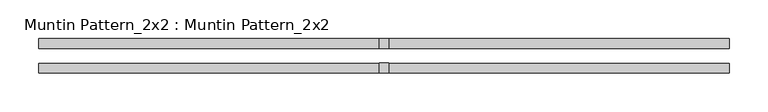
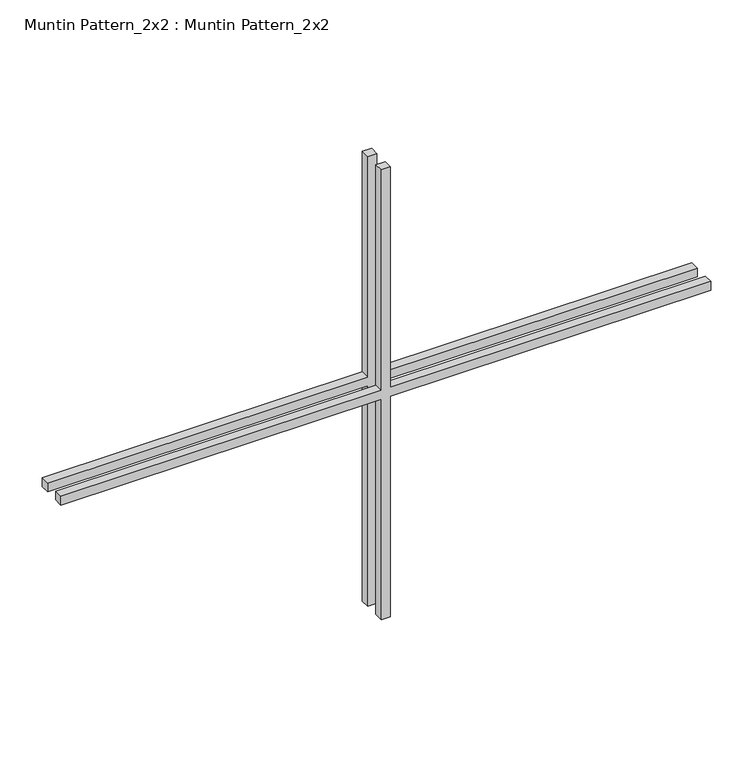
"""IFC4 building model written with IfcOpenShell, lengths in millimetres: proxy geometry, Muntin Pattern_2x2 : Muntin Pattern_2x2."""

import ifcopenshell
import ifcopenshell.guid

model = None  # the IFC model being written
_history = None  # IfcOwnerHistory: only IFC2X3 demands one
_inside = {}  # id of a spatial element -> (the spatial element, [elements in it])
_under = {}  # id of a project, library or spatial element -> (it, [spatial elements below it])
_declared = {}  # id of a project -> (the project, [libraries it declares])
_typed = {}  # id of a type object -> (the type object, [elements of that type])
_made_of = {}  # id of a material, layer set ... -> (it, [elements and type objects made of it])


def new_model(schema):
    """Start an empty IFC model of exactly this schema.

    Asked for "IFC4X3", IfcOpenShell would pick the latest addendum, in which some entities
    have other attributes; the version numbers below select the first issue.
    IFC2X3 requires an IfcOwnerHistory on every rooted entity: one is made here for all.
    """
    global model, _history
    if schema == "IFC4X3":
        model = ifcopenshell.file(schema_version=(4, 3, 0, 0))
    else:
        model = ifcopenshell.file(schema=schema)
    _inside.clear()
    _under.clear()
    _declared.clear()
    _typed.clear()
    _made_of.clear()
    _history = None
    if model.schema == "IFC2X3":
        org = make("IfcOrganization", Name="unknown")
        user = make(
            "IfcPersonAndOrganization",
            ThePerson=make("IfcPerson", FamilyName="unknown"),
            TheOrganization=org,
        )
        app = make(
            "IfcApplication",
            ApplicationDeveloper=org,
            Version="unknown",
            ApplicationFullName="unknown",
            ApplicationIdentifier="unknown",
        )
        _history = make(
            "IfcOwnerHistory",
            OwningUser=user,
            OwningApplication=app,
            ChangeAction="ADDED",
            CreationDate=0,
        )
    return model


def make(cls, **values):
    """One entity of the class cls with the attributes given. An attribute that is None is left unset."""
    return model.create_entity(
        cls, **{name: value for name, value in values.items() if value is not None}
    )


def rooted(cls, **values):
    """An entity with a GlobalId (a new one), such as an element, a storey or a relation."""
    return make(cls, GlobalId=ifcopenshell.guid.new(), OwnerHistory=_history, **values)


def si_unit(unit_type, name, prefix=None):
    """IfcSIUnit, for example si_unit("LENGTHUNIT", "METRE", prefix="MILLI")."""
    return make("IfcSIUnit", UnitType=unit_type, Prefix=prefix, Name=name)


def assignment(units):
    """IfcUnitAssignment: the units of a project."""
    return None if units is None else make("IfcUnitAssignment", Units=units)


def point(xyz):
    """IfcCartesianPoint."""
    return None if xyz is None else make("IfcCartesianPoint", Coordinates=xyz)


def direction(xyz):
    """IfcDirection."""
    return None if xyz is None else make("IfcDirection", DirectionRatios=xyz)


def frame(location, z_axis=None, x_axis=None):
    """IfcAxis2Placement3D, a coordinate frame: its origin and axes. An axis left out is left unset."""
    return make(
        "IfcAxis2Placement3D",
        Location=point(location),
        Axis=direction(z_axis),
        RefDirection=direction(x_axis),
    )


def origin():
    """The frame at (0, 0, 0) with its axes left unset."""
    return frame((0.0, 0.0, 0.0))


def place(relative_to, where):
    """IfcLocalPlacement: puts the frame where relative to a parent placement (None: the world)."""
    return make(
        "IfcLocalPlacement", PlacementRelTo=relative_to, RelativePlacement=where
    )


def context(
    kind, dimensions, precision=None, world=None, true_north=None, identifier=None
):
    """IfcGeometricRepresentationContext, for example the 3D "Model" context."""
    return make(
        "IfcGeometricRepresentationContext",
        ContextIdentifier=identifier,
        ContextType=kind,
        CoordinateSpaceDimension=dimensions,
        Precision=precision,
        WorldCoordinateSystem=world,
        TrueNorth=true_north,
    )


def project(units=None, contexts=None):
    """IfcProject with its units and contexts."""
    return rooted(
        "IfcProject",
        Name="project",
        RepresentationContexts=contexts,
        UnitsInContext=assignment(units),
    )


def spatial(cls, under=None, at=None, **own):
    """A site, building, storey or space (cls), placed at a placement, below another one or the project."""
    s = rooted(cls, ObjectPlacement=at, **own)
    if under is not None:
        _under.setdefault(under.id(), (under, []))[1].append(s)
    return s


def polyline(points):
    """IfcPolyline through the points."""
    return make("IfcPolyline", Points=[point(p) for p in points])


def outline(outer, holes=None, kind="AREA"):
    """IfcArbitraryClosedProfileDef: a profile drawn as a closed curve; with holes, ...WithVoids."""
    if holes is None:
        return make("IfcArbitraryClosedProfileDef", ProfileType=kind, OuterCurve=outer)
    return make(
        "IfcArbitraryProfileDefWithVoids",
        ProfileType=kind,
        OuterCurve=outer,
        InnerCurves=holes,
    )


def extrude(swept, where, along, depth):
    """IfcExtrudedAreaSolid: the profile swept, set in the frame where, extruded along a direction by depth."""
    return make(
        "IfcExtrudedAreaSolid",
        SweptArea=swept,
        Position=where,
        ExtrudedDirection=direction(along),
        Depth=depth,
    )


def shape(context_of_items, identifier, shape_type, items):
    """IfcShapeRepresentation: the items that make up one representation, for example the "Body"."""
    return make(
        "IfcShapeRepresentation",
        ContextOfItems=context_of_items,
        RepresentationIdentifier=identifier,
        RepresentationType=shape_type,
        Items=items,
    )


def source(mapping_origin, context_of_items, identifier, shape_type, items):
    """IfcRepresentationMap: a shape defined once, which mapped items show again and again."""
    return make(
        "IfcRepresentationMap",
        MappingOrigin=mapping_origin,
        MappedRepresentation=shape(context_of_items, identifier, shape_type, items),
    )


def transform(
    local_origin,
    x_axis=None,
    y_axis=None,
    z_axis=None,
    scale=None,
    scale2=None,
    scale3=None,
    uniform=True,
):
    """IfcCartesianTransformationOperator3D, or its non-uniform kind. x_axis, y_axis, z_axis: its Axis1, 2, 3."""
    if uniform:
        return make(
            "IfcCartesianTransformationOperator3D",
            Axis1=direction(x_axis),
            Axis2=direction(y_axis),
            LocalOrigin=point(local_origin),
            Scale=scale,
            Axis3=direction(z_axis),
        )
    return make(
        "IfcCartesianTransformationOperator3DnonUniform",
        Axis1=direction(x_axis),
        Axis2=direction(y_axis),
        LocalOrigin=point(local_origin),
        Scale=scale,
        Axis3=direction(z_axis),
        Scale2=scale2,
        Scale3=scale3,
    )


def mapped(mapping_source, mapping_target):
    """IfcMappedItem: shows the shape of a source again, moved by a transform."""
    return make(
        "IfcMappedItem", MappingSource=mapping_source, MappingTarget=mapping_target
    )


def made_of(thing, what):
    """Note that an element or type object is made of a material, layer set ...; save() writes the relation."""
    if what is not None:
        _made_of.setdefault(what.id(), (what, []))[1].append(thing)
    return thing


def element(
    cls,
    number,
    at=None,
    inside=None,
    cuts=None,
    type_object=None,
    material=None,
    context=None,
    identifier="Body",
    shape_type=None,
    held_by="IfcProductDefinitionShape",
    body=None,
    shapes=None,
    **own,
):
    """One element of the class cls, such as IfcWall. Its Tag is "e" and its number.

    at: its placement. inside: the storey or other place that contains it. cuts: it is an
    opening in that element (IfcRelVoidsElement). A single representation is given by context,
    identifier, shape_type and body (its items); several are given by shapes. held_by: the class
    of the entity that holds the representations. save() writes the other relations.
    """
    e = rooted(cls, Tag="e%d" % number, ObjectPlacement=at, **own)
    if body is not None:
        shapes = [shape(context, identifier, shape_type, body)]
    if shapes is not None:
        e.Representation = make(held_by, Representations=shapes)
    if inside is not None:
        _inside.setdefault(inside.id(), (inside, []))[1].append(e)
    if cuts is not None:
        rooted(
            "IfcRelVoidsElement", RelatingBuildingElement=cuts, RelatedOpeningElement=e
        )
    if type_object is not None:
        _typed.setdefault(type_object.id(), (type_object, []))[1].append(e)
    return made_of(e, material)


def aggregate(whole, parts):
    """IfcRelAggregates: a whole, such as a stair, and the parts it consists of."""
    return rooted("IfcRelAggregates", RelatingObject=whole, RelatedObjects=parts)


def save(model, path):
    """Write the relations noted so far, then the file.

    IfcRelAggregates (storeys below a building ...), IfcRelContainedInSpatialStructure (elements
    in a storey), IfcRelDefinesByType, IfcRelAssociatesMaterial and IfcRelDeclares: one each for
    every whole, place, type object, material and project.
    """
    for whole, parts in _under.values():
        aggregate(whole, parts)
    for where, things in _inside.values():
        rooted(
            "IfcRelContainedInSpatialStructure",
            RelatedElements=things,
            RelatingStructure=where,
        )
    for kind, things in _typed.values():
        rooted("IfcRelDefinesByType", RelatedObjects=things, RelatingType=kind)
    for what, things in _made_of.values():
        rooted("IfcRelAssociatesMaterial", RelatedObjects=things, RelatingMaterial=what)
    for by, libraries in _declared.values():
        rooted("IfcRelDeclares", RelatingContext=by, RelatedDefinitions=libraries)
    model.write(path)


def muntin_pattern_2x2_muntin_pattern_2x2_9281f183(model_context):
    return source(origin(), model_context, "Body", "SweptSolid", [
        extrude(outline(polyline([(331.7875, -6.35), (331.7875, -444.5), (319.0875, -444.5), (319.0875, -6.35), (0.0, -6.35), (0.0, 6.35), (319.0875, 6.35), (319.0875, 444.5), (331.7875, 444.5), (331.7875, 6.35), (650.875, 6.35), (650.875, -6.35), (331.7875, -6.35)])), frame((0.0, 9.525, 0.0), z_axis=(0.0, 1.0, 0.0), x_axis=(0.0, 0.0, 1.0)), (0.0, 0.0, 1.0), 12.7),
        extrude(outline(polyline([(331.7875, -6.35), (331.7875, -444.5), (319.0875, -444.5), (319.0875, -6.35), (0.0, -6.35), (0.0, 6.35), (319.0875, 6.35), (319.0875, 444.5), (331.7875, 444.5), (331.7875, 6.35), (650.875, 6.35), (650.875, -6.35), (331.7875, -6.35)])), frame((0.0, -22.225, 0.0), z_axis=(0.0, 1.0, 0.0), x_axis=(0.0, 0.0, 1.0)), (0.0, 0.0, 1.0), 12.7),
    ])


if __name__ == "__main__":
    model = new_model("IFC4")
    model_context = context("Model", 3, world=origin())
    ifc_project = project(units=[si_unit("LENGTHUNIT", "METRE", prefix="MILLI")], contexts=[model_context])
    site = spatial("IfcSite", under=ifc_project)
    building = spatial("IfcBuilding", under=site)
    placement = place(None, origin())
    muntin_pattern_2x2_muntin_pattern_2x2_shape = muntin_pattern_2x2_muntin_pattern_2x2_9281f183(model_context)
    element("IfcBuildingElementProxy", 1, Name="Muntin Pattern_2x2 : Muntin Pattern_2x2", ObjectType="Muntin Pattern_2x2 : Muntin Pattern_2x2", at=placement, inside=building, context=model_context, shape_type="MappedRepresentation", body=[
        mapped(muntin_pattern_2x2_muntin_pattern_2x2_shape, transform((0.0, 0.0, 0.0), x_axis=(1.0, 0.0, 0.0), y_axis=(0.0, 1.0, 0.0), z_axis=(0.0, 0.0, 1.0))),
    ])
    save(model, "model.ifc")

# Revit data of these elements
# Type "Muntin Pattern_2x2 : Muntin Pattern_2x2"
#   Width [instance default] = 4' - 0"
#   Thickness = 0' - 0 1/2"
#   Height [instance default] = 4' - 0"
#   Distance = 0' - 0 3/4"
#   Interior Material [instance default] = none
#   Exterior Material [instance default] = none
# Element 1 (IfcBuildingElementProxy, "Muntin Pattern_2x2 : Muntin Pattern_2x2")
#   Width = 2' - 11"
#   Height = 2' - 1 5/8"
#   Interior Material = Wood - Stained
#   Exterior Material = Clad - White
#   Materials on its faces: "Clad - White", "Wood - Stained"
# Materials
#   "Clad - White": class "Wood", colour RGB 242 242 238, transparency 0, Cost = 0
#   "Wood - Stained": class "Wood", colour RGB 224 178 126, transparency 0, Cost = 0
